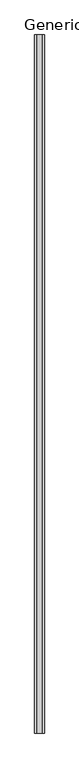
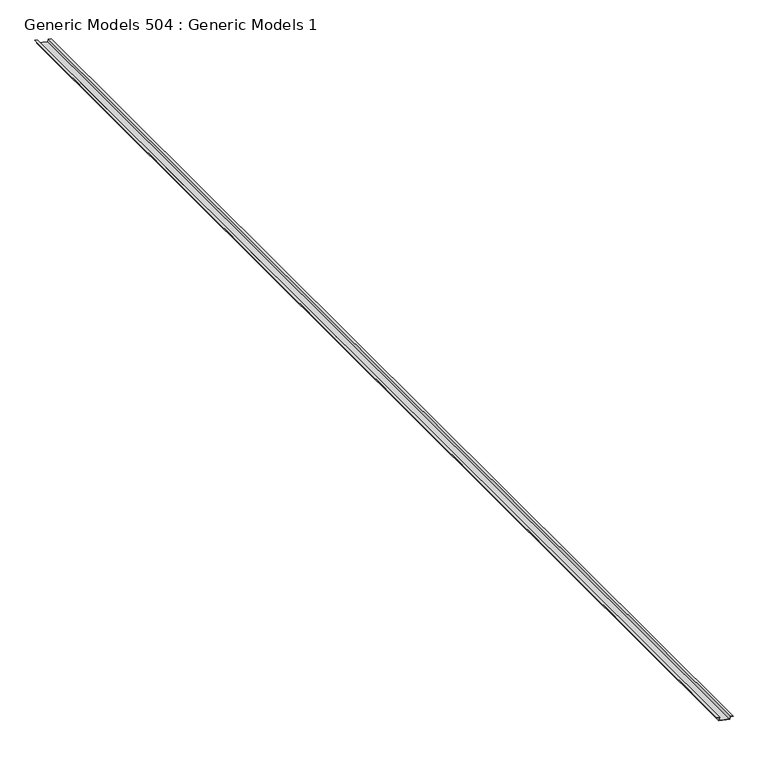
"""IFC4 building model written with IfcOpenShell, lengths in millimetres: proxy geometry, Generic Models 504 : Generic Models 1."""

from ifc_helpers import new_model, si_unit, frame, origin, place, context, project, spatial, polyline, outline, extrude, source, transform, mapped, element, save


def generic_models_504_generic_models_1_86192962(model_context):
    return source(origin(), model_context, "Body", "SweptSolid", [
        extrude(outline(polyline([(129388.9030565, 1929.8860622), (129393.5426114, 1911.3278425), (129375.0613968, 1906.7075389), (129392.926571, 1835.2468423), (129411.4077856, 1839.8671459), (129416.0473405, 1821.3089263), (129414.8152595, 1821.000906), (129410.4837249, 1838.3270447), (129392.0025102, 1833.7067411), (129373.5212956, 1907.6315996), (129392.0025102, 1912.2519032), (129387.6709755, 1929.578042), (129388.9030565, 1929.8860622)])), frame((0.0, 306.6963299, 0.0), z_axis=(0.0, 1.0, 0.0), x_axis=(0.0, 0.0, 1.0)), (0.0, 0.0, 1.0), 7886.7),
    ])


if __name__ == "__main__":
    model = new_model("IFC4")
    model_context = context("Model", 3, world=origin())
    ifc_project = project(units=[si_unit("LENGTHUNIT", "METRE", prefix="MILLI")], contexts=[model_context])
    site = spatial("IfcSite", under=ifc_project)
    building = spatial("IfcBuilding", under=site)
    placement = place(None, origin())
    generic_models_504_generic_models_1_shape = generic_models_504_generic_models_1_86192962(model_context)
    element("IfcBuildingElementProxy", 1, Name="Generic Models 504 : Generic Models 1", ObjectType="Generic Models 504 : Generic Models 1", at=placement, inside=building, context=model_context, shape_type="MappedRepresentation", body=[
        mapped(generic_models_504_generic_models_1_shape, transform((0.0, 0.0, 0.0), x_axis=(1.0, 0.0, 0.0), y_axis=(0.0, 1.0, 0.0), z_axis=(0.0, 0.0, 1.0))),
    ])
    save(model, "model.ifc")

# Revit data of these elements
# Element 1 (IfcBuildingElementProxy, "Generic Models 504 : Generic Models 1")
#   Materials on its faces: "_CONTINUOUS 16 GA. VENTED SOFFIT"
# Materials
#   "_CONTINUOUS 16 GA. VENTED SOFFIT": class "Generic", colour RGB 253 192 103, transparency 0, Cost = 0
